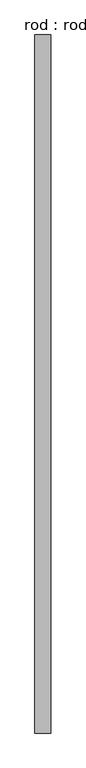
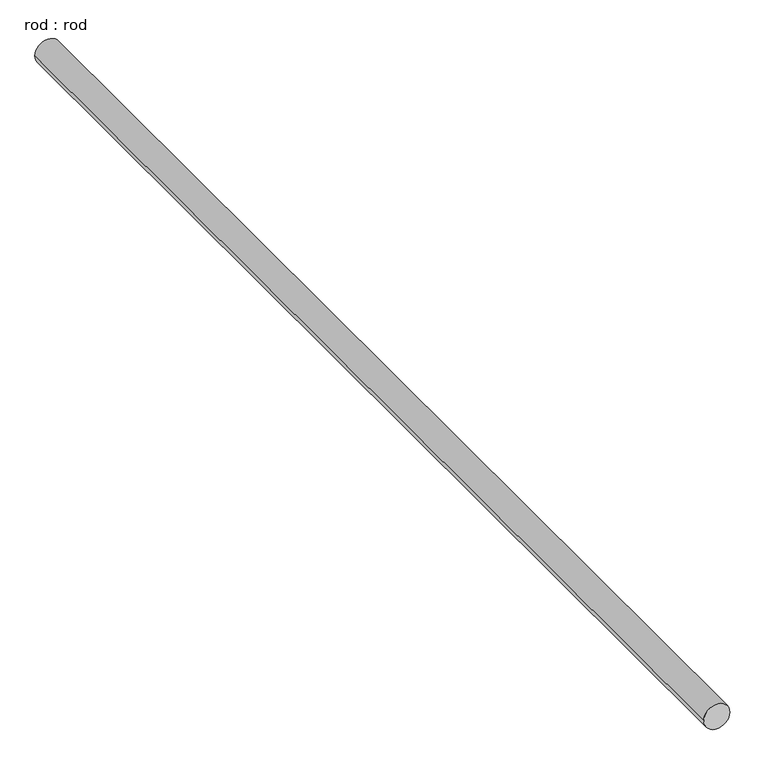
"""IFC4 building model written with IfcOpenShell, lengths in millimetres: proxy geometry, rod : rod."""

from ifc_helpers import new_model, si_unit, point, frame, frame_2d, origin, place, context, project, spatial, circle_curve, trimmed, segment, composite_curve, outline, extrude, source, transform, mapped, element, save


def rod_rod_0f2eb7da(model_context):
    return source(origin(), model_context, "Body", "SweptSolid", [
        extrude(outline(composite_curve([segment(trimmed(circle_curve(frame_2d((0.0108462, 0.0)), 200.0), [point((0.0108462, 200.0))], [point((0.0108462, -200.0))], False, "CARTESIAN"), True, "CONTINUOUS"), segment(trimmed(circle_curve(frame_2d((0.0108462, 0.0)), 200.0), [point((0.0108462, -200.0))], [point((0.0108462, 200.0))], False, "CARTESIAN"), True, "CONTINUOUS")], self_intersect=False)), frame((0.0, -4793.4530847, 0.0), z_axis=(0.0, 1.0, 0.0), x_axis=(0.0, 0.0, 1.0)), (0.0, 0.0, 1.0), 17772.3634001),
    ])


if __name__ == "__main__":
    model = new_model("IFC4")
    model_context = context("Model", 3, world=origin())
    ifc_project = project(units=[si_unit("LENGTHUNIT", "METRE", prefix="MILLI")], contexts=[model_context])
    site = spatial("IfcSite", under=ifc_project)
    building = spatial("IfcBuilding", under=site)
    placement = place(None, origin())
    rod_rod_shape = rod_rod_0f2eb7da(model_context)
    element("IfcBuildingElementProxy", 1, Name="rod : rod", ObjectType="rod : rod", at=placement, inside=building, context=model_context, shape_type="MappedRepresentation", body=[
        mapped(rod_rod_shape, transform((0.0, 0.0, 0.0), x_axis=(1.0, 0.0, 0.0), y_axis=(0.0, 1.0, 0.0), z_axis=(0.0, 0.0, 1.0))),
    ])
    save(model, "model.ifc")

# Revit data of these elements
# Type "rod : rod"
#   Default Elevation = 0
